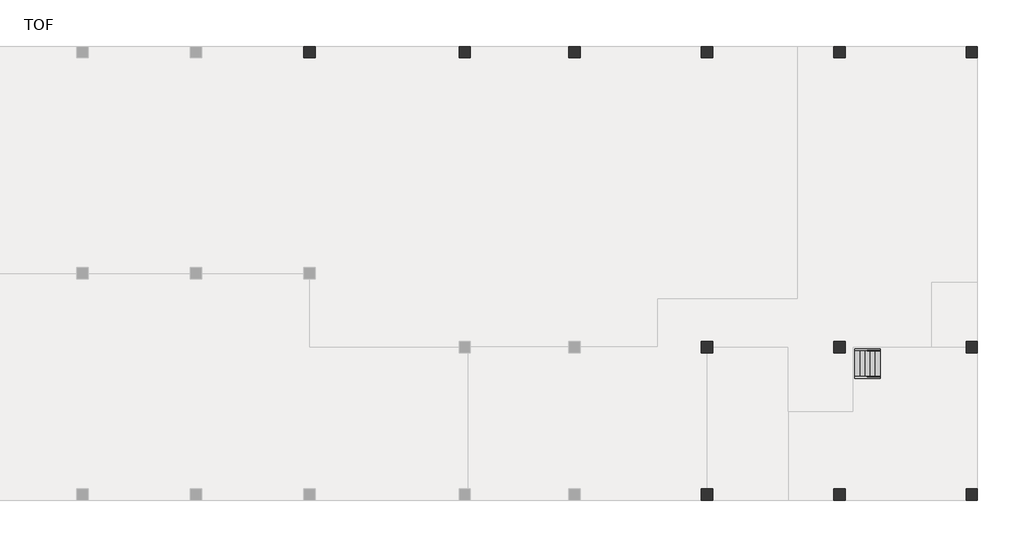
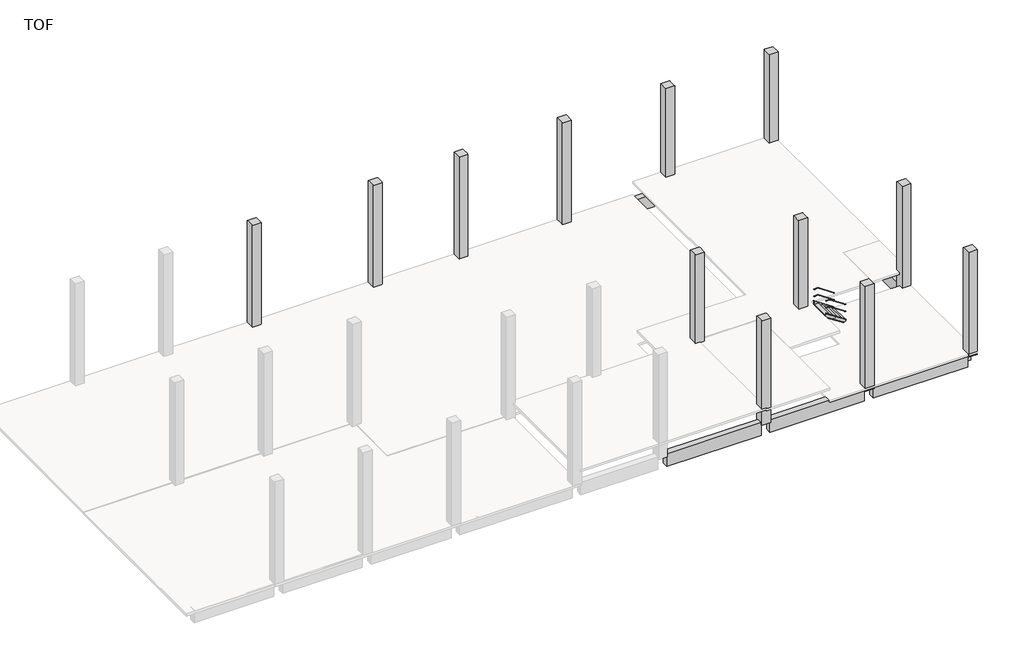
# One storey, part 2 of 2: 12 columns, 11 beams, 2 members, 2 railings, 1 stair flight.
"""IFC4 building model written with IfcOpenShell, lengths in millimetres."""

import ifcopenshell
import ifcopenshell.guid

model = None  # the IFC model being written
_history = None  # IfcOwnerHistory: only IFC2X3 demands one
_inside = {}  # id of a spatial element -> (the spatial element, [elements in it])
_under = {}  # id of a project, library or spatial element -> (it, [spatial elements below it])
_declared = {}  # id of a project -> (the project, [libraries it declares])
_typed = {}  # id of a type object -> (the type object, [elements of that type])
_made_of = {}  # id of a material, layer set ... -> (it, [elements and type objects made of it])


def new_model(schema):
    """Start an empty IFC model of exactly this schema.

    Asked for "IFC4X3", IfcOpenShell would pick the latest addendum, in which some entities
    have other attributes; the version numbers below select the first issue.
    IFC2X3 requires an IfcOwnerHistory on every rooted entity: one is made here for all.
    """
    global model, _history
    if schema == "IFC4X3":
        model = ifcopenshell.file(schema_version=(4, 3, 0, 0))
    else:
        model = ifcopenshell.file(schema=schema)
    _inside.clear()
    _under.clear()
    _declared.clear()
    _typed.clear()
    _made_of.clear()
    _history = None
    if model.schema == "IFC2X3":
        org = make("IfcOrganization", Name="unknown")
        user = make(
            "IfcPersonAndOrganization",
            ThePerson=make("IfcPerson", FamilyName="unknown"),
            TheOrganization=org,
        )
        app = make(
            "IfcApplication",
            ApplicationDeveloper=org,
            Version="unknown",
            ApplicationFullName="unknown",
            ApplicationIdentifier="unknown",
        )
        _history = make(
            "IfcOwnerHistory",
            OwningUser=user,
            OwningApplication=app,
            ChangeAction="ADDED",
            CreationDate=0,
        )
    return model


def make(cls, **values):
    """One entity of the class cls with the attributes given. An attribute that is None is left unset."""
    return model.create_entity(
        cls, **{name: value for name, value in values.items() if value is not None}
    )


def rooted(cls, **values):
    """An entity with a GlobalId (a new one), such as an element, a storey or a relation."""
    return make(cls, GlobalId=ifcopenshell.guid.new(), OwnerHistory=_history, **values)


def si_unit(unit_type, name, prefix=None):
    """IfcSIUnit, for example si_unit("LENGTHUNIT", "METRE", prefix="MILLI")."""
    return make("IfcSIUnit", UnitType=unit_type, Prefix=prefix, Name=name)


def assignment(units):
    """IfcUnitAssignment: the units of a project."""
    return None if units is None else make("IfcUnitAssignment", Units=units)


def point(xyz):
    """IfcCartesianPoint."""
    return None if xyz is None else make("IfcCartesianPoint", Coordinates=xyz)


def direction(xyz):
    """IfcDirection."""
    return None if xyz is None else make("IfcDirection", DirectionRatios=xyz)


def frame(location, z_axis=None, x_axis=None):
    """IfcAxis2Placement3D, a coordinate frame: its origin and axes. An axis left out is left unset."""
    return make(
        "IfcAxis2Placement3D",
        Location=point(location),
        Axis=direction(z_axis),
        RefDirection=direction(x_axis),
    )


def origin():
    """The frame at (0, 0, 0) with its axes left unset."""
    return frame((0.0, 0.0, 0.0))


def place(relative_to, where):
    """IfcLocalPlacement: puts the frame where relative to a parent placement (None: the world)."""
    return make(
        "IfcLocalPlacement", PlacementRelTo=relative_to, RelativePlacement=where
    )


def context(
    kind, dimensions, precision=None, world=None, true_north=None, identifier=None
):
    """IfcGeometricRepresentationContext, for example the 3D "Model" context."""
    return make(
        "IfcGeometricRepresentationContext",
        ContextIdentifier=identifier,
        ContextType=kind,
        CoordinateSpaceDimension=dimensions,
        Precision=precision,
        WorldCoordinateSystem=world,
        TrueNorth=true_north,
    )


def project(units=None, contexts=None):
    """IfcProject with its units and contexts."""
    return rooted(
        "IfcProject",
        Name="project",
        RepresentationContexts=contexts,
        UnitsInContext=assignment(units),
    )


def spatial(cls, under=None, at=None, **own):
    """A site, building, storey or space (cls), placed at a placement, below another one or the project."""
    s = rooted(cls, ObjectPlacement=at, **own)
    if under is not None:
        _under.setdefault(under.id(), (under, []))[1].append(s)
    return s


def polyline(points):
    """IfcPolyline through the points."""
    return make("IfcPolyline", Points=[point(p) for p in points])


def circle_curve(where, radius):
    """IfcCircle in the frame where."""
    return make("IfcCircle", Position=where, Radius=radius)


def ellipse_curve(where, semi_axis1, semi_axis2):
    """IfcEllipse in the frame where."""
    return make(
        "IfcEllipse", Position=where, SemiAxis1=semi_axis1, SemiAxis2=semi_axis2
    )


def outline(outer, holes=None, kind="AREA"):
    """IfcArbitraryClosedProfileDef: a profile drawn as a closed curve; with holes, ...WithVoids."""
    if holes is None:
        return make("IfcArbitraryClosedProfileDef", ProfileType=kind, OuterCurve=outer)
    return make(
        "IfcArbitraryProfileDefWithVoids",
        ProfileType=kind,
        OuterCurve=outer,
        InnerCurves=holes,
    )


def extrude(swept, where, along, depth):
    """IfcExtrudedAreaSolid: the profile swept, set in the frame where, extruded along a direction by depth."""
    return make(
        "IfcExtrudedAreaSolid",
        SweptArea=swept,
        Position=where,
        ExtrudedDirection=direction(along),
        Depth=depth,
    )


def faces_of(points, faces, orient=None, outer=None):
    """IfcFace entities. A face is a list of loops; a loop is a list of indices into points, from 0.

    orient and outer hold one flag for each loop. By default every Orientation is true, the
    first loop of a face is its IfcFaceOuterBound and the others are IfcFaceBound.
    """
    made = []
    for i, loops in enumerate(faces):
        bounds = []
        for j, loop in enumerate(loops):
            is_outer = j == 0 if outer is None else outer[i][j]
            bounds.append(
                make(
                    "IfcFaceOuterBound" if is_outer else "IfcFaceBound",
                    Bound=make("IfcPolyLoop", Polygon=[points[k] for k in loop]),
                    Orientation=True if orient is None else orient[i][j],
                )
            )
        made.append(make("IfcFace", Bounds=bounds))
    return made


def faceted_brep(points, faces, orient=None, outer=None, voids=None):
    """IfcFacetedBrep: a solid bounded by flat faces; with voids (closed shells), ...WithVoids."""
    shared = [point(p) for p in points]
    hull = make("IfcClosedShell", CfsFaces=faces_of(shared, faces, orient, outer))
    if voids is None:
        return make("IfcFacetedBrep", Outer=hull)
    return make(
        "IfcFacetedBrepWithVoids",
        Outer=hull,
        Voids=[
            make(cls, CfsFaces=faces_of(shared, fs, o, b)) for cls, fs, o, b in voids
        ],
    )


def shape(context_of_items, identifier, shape_type, items):
    """IfcShapeRepresentation: the items that make up one representation, for example the "Body"."""
    return make(
        "IfcShapeRepresentation",
        ContextOfItems=context_of_items,
        RepresentationIdentifier=identifier,
        RepresentationType=shape_type,
        Items=items,
    )


def source(mapping_origin, context_of_items, identifier, shape_type, items):
    """IfcRepresentationMap: a shape defined once, which mapped items show again and again."""
    return make(
        "IfcRepresentationMap",
        MappingOrigin=mapping_origin,
        MappedRepresentation=shape(context_of_items, identifier, shape_type, items),
    )


def transform(
    local_origin,
    x_axis=None,
    y_axis=None,
    z_axis=None,
    scale=None,
    scale2=None,
    scale3=None,
    uniform=True,
):
    """IfcCartesianTransformationOperator3D, or its non-uniform kind. x_axis, y_axis, z_axis: its Axis1, 2, 3."""
    if uniform:
        return make(
            "IfcCartesianTransformationOperator3D",
            Axis1=direction(x_axis),
            Axis2=direction(y_axis),
            LocalOrigin=point(local_origin),
            Scale=scale,
            Axis3=direction(z_axis),
        )
    return make(
        "IfcCartesianTransformationOperator3DnonUniform",
        Axis1=direction(x_axis),
        Axis2=direction(y_axis),
        LocalOrigin=point(local_origin),
        Scale=scale,
        Axis3=direction(z_axis),
        Scale2=scale2,
        Scale3=scale3,
    )


def mapped(mapping_source, mapping_target):
    """IfcMappedItem: shows the shape of a source again, moved by a transform."""
    return make(
        "IfcMappedItem", MappingSource=mapping_source, MappingTarget=mapping_target
    )


def made_of(thing, what):
    """Note that an element or type object is made of a material, layer set ...; save() writes the relation."""
    if what is not None:
        _made_of.setdefault(what.id(), (what, []))[1].append(thing)
    return thing


def element(
    cls,
    number,
    at=None,
    inside=None,
    cuts=None,
    type_object=None,
    material=None,
    context=None,
    identifier="Body",
    shape_type=None,
    held_by="IfcProductDefinitionShape",
    body=None,
    shapes=None,
    **own,
):
    """One element of the class cls, such as IfcWall. Its Tag is "e" and its number.

    at: its placement. inside: the storey or other place that contains it. cuts: it is an
    opening in that element (IfcRelVoidsElement). A single representation is given by context,
    identifier, shape_type and body (its items); several are given by shapes. held_by: the class
    of the entity that holds the representations. save() writes the other relations.
    """
    e = rooted(cls, Tag="e%d" % number, ObjectPlacement=at, **own)
    if body is not None:
        shapes = [shape(context, identifier, shape_type, body)]
    if shapes is not None:
        e.Representation = make(held_by, Representations=shapes)
    if inside is not None:
        _inside.setdefault(inside.id(), (inside, []))[1].append(e)
    if cuts is not None:
        rooted(
            "IfcRelVoidsElement", RelatingBuildingElement=cuts, RelatedOpeningElement=e
        )
    if type_object is not None:
        _typed.setdefault(type_object.id(), (type_object, []))[1].append(e)
    return made_of(e, material)


def aggregate(whole, parts):
    """IfcRelAggregates: a whole, such as a stair, and the parts it consists of."""
    return rooted("IfcRelAggregates", RelatingObject=whole, RelatedObjects=parts)


def save(model, path):
    """Write the relations noted so far, then the file.

    IfcRelAggregates (storeys below a building ...), IfcRelContainedInSpatialStructure (elements
    in a storey), IfcRelDefinesByType, IfcRelAssociatesMaterial and IfcRelDeclares: one each for
    every whole, place, type object, material and project.
    """
    for whole, parts in _under.values():
        aggregate(whole, parts)
    for where, things in _inside.values():
        rooted(
            "IfcRelContainedInSpatialStructure",
            RelatedElements=things,
            RelatingStructure=where,
        )
    for kind, things in _typed.values():
        rooted("IfcRelDefinesByType", RelatedObjects=things, RelatingType=kind)
    for what, things in _made_of.values():
        rooted("IfcRelAssociatesMaterial", RelatedObjects=things, RelatingMaterial=what)
    for by, libraries in _declared.values():
        rooted("IfcRelDeclares", RelatingContext=by, RelatedDefinitions=libraries)
    model.write(path)


def plane_surface(at):
    """IfcPlane: the flat surface through the origin of the frame at, square to its z axis."""
    return make("IfcPlane", Position=at)


def cylinder_surface(at, radius):
    """IfcCylindricalSurface: all points at the distance radius from the z axis of the frame at."""
    return make("IfcCylindricalSurface", Position=at, Radius=radius)


def advanced_brep(points, edges, surfaces, faces):
    """IfcAdvancedBrep: a solid bounded by faces that lie on surfaces and meet in shared edges.

    An edge is (start, end): straight between two places in points (the first is 0);
    or (start, end, curve); or (start, end, curve, False) where it runs against its curve.
    A face is (place in surfaces, loops), or (place, loops, False) where it looks against
    its surface's normal. A loop lists edges by number (the first is 1), with a minus sign
    where the edge is run from its end to its start. The first loop is the outer one.
    """
    corners = [point(p) for p in points]
    vertices = [make("IfcVertexPoint", VertexGeometry=c) for c in corners]
    made = []
    for start, end, *more in edges:
        made.append(
            make(
                "IfcEdgeCurve",
                EdgeStart=vertices[start],
                EdgeEnd=vertices[end],
                EdgeGeometry=more[0] if more else make("IfcPolyline", Points=[corners[start], corners[end]]),
                SameSense=more[1] if len(more) > 1 else True,
            )
        )
    hull = []
    for where, loops, *sense in faces:
        bounds = []
        for j, loop in enumerate(loops):
            ring = [make("IfcOrientedEdge", EdgeElement=made[abs(k) - 1], Orientation=k > 0) for k in loop]
            bounds.append(
                make(
                    "IfcFaceOuterBound" if j == 0 else "IfcFaceBound",
                    Bound=make("IfcEdgeLoop", EdgeList=ring),
                    Orientation=True,
                )
            )
        hull.append(make("IfcAdvancedFace", Bounds=bounds, FaceSurface=surfaces[where], SameSense=sense[0] if sense else True))
    return make("IfcAdvancedBrep", Outer=make("IfcClosedShell", CfsFaces=hull))


def railing_36ed9c91(model_context):
    return source(origin(), model_context, "Body", "AdvancedBrep", [
        advanced_brep(
        [(48078.2332408, 8219.6306666, 910.5875748), (48078.2332408, 8249.6306666, 910.5875748), (46993.7216539, 8219.6306666, 1627.8571429), (46993.7216539, 8249.6306666, 1627.8571429), (46728.2332408, 8219.6306666, 1627.8571429), (46728.2332408, 8249.6306666, 1627.8571429)],
        [
            (0, 1, ellipse_curve(frame((48078.2332408, 8234.6306666, 910.5875748), z_axis=(1.0, 0.0, 0.0), x_axis=(0.0, 0.0, -1.0)), 17.9838538, 15.0)),
            (1, 0, ellipse_curve(frame((48078.2332408, 8234.6306666, 910.5875748), z_axis=(1.0, 0.0, 0.0), x_axis=(0.0, 0.0, -1.0)), 17.9838538, 15.0)),
            (0, 2),
            (2, 3, ellipse_curve(frame((46993.7216539, 8234.6306666, 1627.8571429), z_axis=(0.9576224501515418, 0.0, -0.28802646226650325), x_axis=(-0.288026462266502, 0.0, -0.9576224501515423)), 15.6637932, 15.0)),
            (3, 1),
            (3, 2, ellipse_curve(frame((46993.7216539, 8234.6306666, 1627.8571429), z_axis=(0.9576224501515418, 0.0, -0.28802646226650325), x_axis=(-0.288026462266502, 0.0, -0.9576224501515423)), 15.6637932, 15.0)),
            (4, 5, circle_curve(frame((46728.2332408, 8234.6306666, 1627.8571429), z_axis=(-1.0, 0.0, 0.0), x_axis=(0.0, 1.0, 0.0)), 15.0)),
            (5, 4, circle_curve(frame((46728.2332408, 8234.6306666, 1627.8571429), z_axis=(-1.0, 0.0, 0.0), x_axis=(0.0, 1.0, 0.0)), 15.0)),
            (2, 4),
            (5, 3),
        ],
        [
            plane_surface(frame((48078.2332408, 8234.6306666, 928.5714286), z_axis=(1.0, 0.0, 0.0), x_axis=(0.0, -1.0, 0.0))),
            cylinder_surface(frame((48069.9586226, 8234.6306666, 916.0602059), z_axis=(0.8340815140684851, 0.0, -0.5516412130082591), x_axis=(0.0, 1.0, 0.0)), 15.0),
            plane_surface(frame((46728.2332408, 8234.6306666, 1642.8571429), z_axis=(-1.0, 0.0, 0.0), x_axis=(0.0, -1.0, 0.0))),
            cylinder_surface(frame((46998.2332408, 8234.6306666, 1627.8571429), z_axis=(1.0, 0.0, 0.0), x_axis=(0.0, 1.0, 0.0)), 15.0),
        ],
        [
            (0, [[1, 2]]),
            (1, [[-1, 3, 4, 5]]),
            (1, [[-2, -5, 6, -3]]),
            (2, [[7, 8]]),
            (3, [[-4, 9, -8, 10]]),
            (3, [[-6, -10, -7, -9]]),
        ],
    ),
        advanced_brep(
        [(48078.2332408, 8219.6306666, 1410.5875748), (48078.2332408, 8249.6306666, 1410.5875748), (46993.7216539, 8219.6306666, 2127.8571429), (46993.7216539, 8249.6306666, 2127.8571429), (46728.2332408, 8219.6306666, 2127.8571429), (46728.2332408, 8249.6306666, 2127.8571429)],
        [
            (0, 1, ellipse_curve(frame((48078.2332408, 8234.6306666, 1410.5875748), z_axis=(1.0, 0.0, 0.0), x_axis=(0.0, 0.0, -1.0)), 17.9838538, 15.0)),
            (1, 0, ellipse_curve(frame((48078.2332408, 8234.6306666, 1410.5875748), z_axis=(1.0, 0.0, 0.0), x_axis=(0.0, 0.0, -1.0)), 17.9838538, 15.0)),
            (0, 2),
            (2, 3, ellipse_curve(frame((46993.7216539, 8234.6306666, 2127.8571429), z_axis=(0.9576224501515418, 0.0, -0.28802646226650325), x_axis=(-0.288026462266502, 0.0, -0.9576224501515423)), 15.6637932, 15.0)),
            (3, 1),
            (3, 2, ellipse_curve(frame((46993.7216539, 8234.6306666, 2127.8571429), z_axis=(0.9576224501515418, 0.0, -0.28802646226650325), x_axis=(-0.288026462266502, 0.0, -0.9576224501515423)), 15.6637932, 15.0)),
            (4, 5, circle_curve(frame((46728.2332408, 8234.6306666, 2127.8571429), z_axis=(-1.0, 0.0, 0.0), x_axis=(0.0, 1.0, 0.0)), 15.0)),
            (5, 4, circle_curve(frame((46728.2332408, 8234.6306666, 2127.8571429), z_axis=(-1.0, 0.0, 0.0), x_axis=(0.0, 1.0, 0.0)), 15.0)),
            (2, 4),
            (5, 3),
        ],
        [
            plane_surface(frame((48078.2332408, 8234.6306666, 1428.5714286), z_axis=(1.0, 0.0, 0.0), x_axis=(0.0, -1.0, 0.0))),
            cylinder_surface(frame((48069.9586226, 8234.6306666, 1416.0602059), z_axis=(0.8340815140684851, 0.0, -0.5516412130082591), x_axis=(0.0, 1.0, 0.0)), 15.0),
            plane_surface(frame((46728.2332408, 8234.6306666, 2142.8571429), z_axis=(-1.0, 0.0, 0.0), x_axis=(0.0, -1.0, 0.0))),
            cylinder_surface(frame((46998.2332408, 8234.6306666, 2127.8571429), z_axis=(1.0, 0.0, 0.0), x_axis=(0.0, 1.0, 0.0)), 15.0),
        ],
        [
            (0, [[1, 2]]),
            (1, [[-1, 3, 4, 5]]),
            (1, [[-2, -5, 6, -3]]),
            (2, [[7, 8]]),
            (3, [[-4, 9, -8, 10]]),
            (3, [[-6, -10, -7, -9]]),
        ],
    ),
    ])


def railing_d88b3958(model_context):
    return source(origin(), model_context, "Body", "AdvancedBrep", [
        advanced_brep(
        [(48078.2332408, 6875.4306666, 910.5875748), (48078.2332408, 6845.4306666, 910.5875748), (46993.7216539, 6875.4306666, 1627.8571429), (46993.7216539, 6845.4306666, 1627.8571429), (46728.2332408, 6875.4306666, 1627.8571429), (46728.2332408, 6845.4306666, 1627.8571429)],
        [
            (0, 1, ellipse_curve(frame((48078.2332408, 6860.4306666, 910.5875748), z_axis=(1.0, 0.0, 0.0), x_axis=(0.0, 0.0, -1.0)), 17.9838538, 15.0)),
            (1, 0, ellipse_curve(frame((48078.2332408, 6860.4306666, 910.5875748), z_axis=(1.0, 0.0, 0.0), x_axis=(0.0, 0.0, -1.0)), 17.9838538, 15.0)),
            (0, 2),
            (2, 3, ellipse_curve(frame((46993.7216539, 6860.4306666, 1627.8571429), z_axis=(0.9576224501515418, 0.0, -0.28802646226650325), x_axis=(-0.288026462266502, 0.0, -0.9576224501515423)), 15.6637932, 15.0)),
            (3, 1),
            (3, 2, ellipse_curve(frame((46993.7216539, 6860.4306666, 1627.8571429), z_axis=(0.9576224501515418, 0.0, -0.28802646226650325), x_axis=(-0.288026462266502, 0.0, -0.9576224501515423)), 15.6637932, 15.0)),
            (4, 5, circle_curve(frame((46728.2332408, 6860.4306666, 1627.8571429), z_axis=(-1.0, 0.0, 0.0), x_axis=(0.0, -1.0, 0.0)), 15.0)),
            (5, 4, circle_curve(frame((46728.2332408, 6860.4306666, 1627.8571429), z_axis=(-1.0, 0.0, 0.0), x_axis=(0.0, -1.0, 0.0)), 15.0)),
            (2, 4),
            (5, 3),
        ],
        [
            plane_surface(frame((48078.2332408, 6860.4306666, 928.5714286), z_axis=(1.0, 0.0, 0.0), x_axis=(0.0, -1.0, 0.0))),
            cylinder_surface(frame((48069.9586226, 6860.4306666, 916.0602059), z_axis=(0.8340815140684851, 0.0, -0.5516412130082591), x_axis=(0.0, -1.0, 0.0)), 15.0),
            plane_surface(frame((46728.2332408, 6860.4306666, 1642.8571429), z_axis=(-1.0, 0.0, 0.0), x_axis=(0.0, -1.0, 0.0))),
            cylinder_surface(frame((46998.2332408, 6860.4306666, 1627.8571429), z_axis=(1.0, 0.0, 0.0), x_axis=(0.0, -1.0, 0.0)), 15.0),
        ],
        [
            (0, [[1, 2]]),
            (1, [[-1, 3, 4, 5]]),
            (1, [[-2, -5, 6, -3]]),
            (2, [[7, 8]]),
            (3, [[-4, 9, -8, 10]]),
            (3, [[-6, -10, -7, -9]]),
        ],
    ),
        advanced_brep(
        [(48078.2332408, 6875.4306666, 1410.5875748), (48078.2332408, 6845.4306666, 1410.5875748), (46993.7216539, 6875.4306666, 2127.8571429), (46993.7216539, 6845.4306666, 2127.8571429), (46728.2332408, 6875.4306666, 2127.8571429), (46728.2332408, 6845.4306666, 2127.8571429)],
        [
            (0, 1, ellipse_curve(frame((48078.2332408, 6860.4306666, 1410.5875748), z_axis=(1.0, 0.0, 0.0), x_axis=(0.0, 0.0, -1.0)), 17.9838538, 15.0)),
            (1, 0, ellipse_curve(frame((48078.2332408, 6860.4306666, 1410.5875748), z_axis=(1.0, 0.0, 0.0), x_axis=(0.0, 0.0, -1.0)), 17.9838538, 15.0)),
            (0, 2),
            (2, 3, ellipse_curve(frame((46993.7216539, 6860.4306666, 2127.8571429), z_axis=(0.9576224501515418, 0.0, -0.28802646226650325), x_axis=(-0.288026462266502, 0.0, -0.9576224501515423)), 15.6637932, 15.0)),
            (3, 1),
            (3, 2, ellipse_curve(frame((46993.7216539, 6860.4306666, 2127.8571429), z_axis=(0.9576224501515418, 0.0, -0.28802646226650325), x_axis=(-0.288026462266502, 0.0, -0.9576224501515423)), 15.6637932, 15.0)),
            (4, 5, circle_curve(frame((46728.2332408, 6860.4306666, 2127.8571429), z_axis=(-1.0, 0.0, 0.0), x_axis=(0.0, -1.0, 0.0)), 15.0)),
            (5, 4, circle_curve(frame((46728.2332408, 6860.4306666, 2127.8571429), z_axis=(-1.0, 0.0, 0.0), x_axis=(0.0, -1.0, 0.0)), 15.0)),
            (2, 4),
            (5, 3),
        ],
        [
            plane_surface(frame((48078.2332408, 6860.4306666, 1428.5714286), z_axis=(1.0, 0.0, 0.0), x_axis=(0.0, -1.0, 0.0))),
            cylinder_surface(frame((48069.9586226, 6860.4306666, 1416.0602059), z_axis=(0.8340815140684851, 0.0, -0.5516412130082591), x_axis=(0.0, -1.0, 0.0)), 15.0),
            plane_surface(frame((46728.2332408, 6860.4306666, 2142.8571429), z_axis=(-1.0, 0.0, 0.0), x_axis=(0.0, -1.0, 0.0))),
            cylinder_surface(frame((46998.2332408, 6860.4306666, 2127.8571429), z_axis=(1.0, 0.0, 0.0), x_axis=(0.0, -1.0, 0.0)), 15.0),
        ],
        [
            (0, [[1, 2]]),
            (1, [[-1, 3, 4, 5]]),
            (1, [[-2, -5, 6, -3]]),
            (2, [[7, 8]]),
            (3, [[-4, 9, -8, 10]]),
            (3, [[-6, -10, -7, -9]]),
        ],
    ),
    ])


def stair_flight_4e27faa5(model_context):
    return source(origin(), model_context, "Body", "SweptSolid", [
        extrude(outline(polyline([(47808.2332408, 6860.0306666), (47808.2332408, 8235.0306666), (48078.2332408, 8235.0306666), (48078.2332408, 6860.0306666), (47808.2332408, 6860.0306666)])), frame((0.0, 0.0, 296.5714286), z_axis=(0.0, 0.0, 1.0), x_axis=(1.0, 0.0, 0.0)), (0.0, 0.0, 1.0), 32.0),
        extrude(outline(polyline([(47538.2332408, 6860.0306666), (47538.2332408, 8235.0306666), (47808.2332408, 8235.0306666), (47808.2332408, 6860.0306666), (47538.2332408, 6860.0306666)])), frame((0.0, 0.0, 475.1428571), z_axis=(0.0, 0.0, 1.0), x_axis=(1.0, 0.0, 0.0)), (0.0, 0.0, 1.0), 32.0),
        extrude(outline(polyline([(47268.2332408, 6860.0306666), (47268.2332408, 8235.0306666), (47538.2332408, 8235.0306666), (47538.2332408, 6860.0306666), (47268.2332408, 6860.0306666)])), frame((0.0, 0.0, 653.7142857), z_axis=(0.0, 0.0, 1.0), x_axis=(1.0, 0.0, 0.0)), (0.0, 0.0, 1.0), 32.0),
        extrude(outline(polyline([(46998.2332408, 6860.0306666), (46998.2332408, 8235.0306666), (47268.2332408, 8235.0306666), (47268.2332408, 6860.0306666), (46998.2332408, 6860.0306666)])), frame((0.0, 0.0, 832.2857143), z_axis=(0.0, 0.0, 1.0), x_axis=(1.0, 0.0, 0.0)), (0.0, 0.0, 1.0), 32.0),
        extrude(outline(polyline([(46728.2332408, 6860.0306666), (46728.2332408, 8235.0306666), (46998.2332408, 8235.0306666), (46998.2332408, 6860.0306666), (46728.2332408, 6860.0306666)])), frame((0.0, 0.0, 1010.8571429), z_axis=(0.0, 0.0, 1.0), x_axis=(1.0, 0.0, 0.0)), (0.0, 0.0, 1.0), 32.0),
    ])


model = new_model("IFC4")

# Units and contexts
model_context = context("Model", 3, world=origin())
ifc_project = project(units=[si_unit("LENGTHUNIT", "METRE", prefix="MILLI")], contexts=[model_context])

# Site, building, storey
site = spatial("IfcSite", under=ifc_project)
building = spatial("IfcBuilding", under=site)
storey = spatial("IfcBuildingStorey", under=building, Name="TOF", Elevation=150.0)

# Beams
placement = place(None, origin())
element("IfcBeam", 1, ObjectType="RC Beam_Rectangular : H_SB_ACB_B400xH900", at=placement, inside=storey, context=model_context, shape_type="SweptSolid", body=[
    extrude(outline(polyline([(52724.7, 23716.5208589), (53124.7, 23716.5208589), (53124.7, 18966.5208589), (52724.7, 18966.5208589), (52724.7, 23716.5208589)])), frame((0.0, 0.0, -750.0), z_axis=(0.0, 0.0, 1.0), x_axis=(1.0, 0.0, 0.0)), (0.0, 0.0, 1.0), 900.0),
    extrude(outline(polyline([(53124.7, 8716.5208589), (52724.7, 8716.5208589), (52724.7, 18366.5208589), (53124.7, 18366.5208589), (53124.7, 8716.5208589)])), frame((0.0, 0.0, -750.0), z_axis=(0.0, 0.0, 1.0), x_axis=(1.0, 0.0, 0.0)), (0.0, 0.0, 1.0), 900.0),
])
element("IfcBeam", 2, ObjectType="RC Beam_Rectangular : H_SB_ACB_B400xH900", at=placement, inside=storey, context=model_context, shape_type="SweptSolid", body=[
    extrude(outline(polyline([(52724.7, 8116.5208589), (53124.7, 8116.5208589), (53124.7, 916.5208589), (52724.7, 916.5208589), (52724.7, 8116.5208589)])), frame((0.0, 0.0, -750.0), z_axis=(0.0, 0.0, 1.0), x_axis=(1.0, 0.0, 0.0)), (0.0, 0.0, 1.0), 900.0),
])
element("IfcBeam", 3, ObjectType="RC Beam_Rectangular : H_SB_ACB_B400xH900", at=placement, inside=storey, context=model_context, shape_type="SweptSolid", body=[
    extrude(outline(polyline([(12224.7, 23816.5208589), (12224.7, 24216.5208589), (17624.7, 24216.5208589), (17624.7, 23816.5208589), (12224.7, 23816.5208589)])), frame((0.0, 0.0, -750.0), z_axis=(0.0, 0.0, 1.0), x_axis=(1.0, 0.0, 0.0)), (0.0, 0.0, 1.0), 900.0),
])
element("IfcBeam", 4, ObjectType="RC Beam_Rectangular : H_SB_ACB_B400xH900", at=placement, inside=storey, context=model_context, shape_type="SweptSolid", body=[
    extrude(outline(polyline([(18224.7, 23816.5208589), (18224.7, 24216.5208589), (25824.7, 24216.5208589), (25824.7, 23816.5208589), (18224.7, 23816.5208589)])), frame((0.0, 0.0, -750.0), z_axis=(0.0, 0.0, 1.0), x_axis=(1.0, 0.0, 0.0)), (0.0, 0.0, 1.0), 900.0),
])
element("IfcBeam", 5, ObjectType="RC Beam_Rectangular : H_SB_ACB_B400xH900", at=placement, inside=storey, context=model_context, shape_type="SweptSolid", body=[
    extrude(outline(polyline([(26424.7, 23816.5208589), (26424.7, 24216.5208589), (31624.7, 24216.5208589), (31624.7, 23816.5208589), (26424.7, 23816.5208589)])), frame((0.0, 0.0, -750.0), z_axis=(0.0, 0.0, 1.0), x_axis=(1.0, 0.0, 0.0)), (0.0, 0.0, 1.0), 900.0),
])
element("IfcBeam", 6, ObjectType="RC Beam_Rectangular : H_SB_ACB_B400xH900", at=placement, inside=storey, context=model_context, shape_type="SweptSolid", body=[
    extrude(outline(polyline([(32224.7, 23816.5208589), (32224.7, 24216.5208589), (38624.7, 24216.5208589), (38624.7, 23816.5208589), (32224.7, 23816.5208589)])), frame((0.0, 0.0, -750.0), z_axis=(0.0, 0.0, 1.0), x_axis=(1.0, 0.0, 0.0)), (0.0, 0.0, 1.0), 900.0),
])
element("IfcBeam", 7, ObjectType="RC Beam_Rectangular : H_SB_ACB_B400xH900", at=placement, inside=storey, context=model_context, shape_type="SweptSolid", body=[
    extrude(outline(polyline([(39224.7, 23816.5208589), (39224.7, 24216.5208589), (45624.7, 24216.5208589), (45624.7, 23816.5208589), (39224.7, 23816.5208589)])), frame((0.0, 0.0, -750.0), z_axis=(0.0, 0.0, 1.0), x_axis=(1.0, 0.0, 0.0)), (0.0, 0.0, 1.0), 900.0),
])
element("IfcBeam", 8, ObjectType="RC Beam_Rectangular : H_SB_ACB_B400xH900", at=placement, inside=storey, context=model_context, shape_type="SweptSolid", body=[
    extrude(outline(polyline([(46224.7, 23816.5208589), (46224.7, 24216.5208589), (52624.7, 24216.5208589), (52624.7, 23816.5208589), (46224.7, 23816.5208589)])), frame((0.0, 0.0, -750.0), z_axis=(0.0, 0.0, 1.0), x_axis=(1.0, 0.0, 0.0)), (0.0, 0.0, 1.0), 900.0),
])
element("IfcBeam", 9, ObjectType="RC Beam_Rectangular : H_SB_ACB_B400xH900", at=placement, inside=storey, context=model_context, shape_type="SweptSolid", body=[
    extrude(outline(polyline([(32224.7, 416.5208589), (32224.7, 816.5208589), (38624.7, 816.5208589), (38624.7, 416.5208589), (32224.7, 416.5208589)])), frame((0.0, 0.0, -750.0), z_axis=(0.0, 0.0, 1.0), x_axis=(1.0, 0.0, 0.0)), (0.0, 0.0, 1.0), 900.0),
])
element("IfcBeam", 10, ObjectType="RC Beam_Rectangular : H_SB_ACB_B400xH900", at=placement, inside=storey, context=model_context, shape_type="SweptSolid", body=[
    extrude(outline(polyline([(39224.7, 416.5208589), (39224.7, 816.5208589), (45624.7, 816.5208589), (45624.7, 416.5208589), (39224.7, 416.5208589)])), frame((0.0, 0.0, -750.0), z_axis=(0.0, 0.0, 1.0), x_axis=(1.0, 0.0, 0.0)), (0.0, 0.0, 1.0), 900.0),
])
element("IfcBeam", 11, ObjectType="RC Beam_Rectangular : H_SB_ACB_B400xH900", at=placement, inside=storey, context=model_context, shape_type="SweptSolid", body=[
    extrude(outline(polyline([(46224.7, 416.5208589), (46224.7, 816.5208589), (52624.7, 816.5208589), (52624.7, 416.5208589), (46224.7, 416.5208589)])), frame((0.0, 0.0, -750.0), z_axis=(0.0, 0.0, 1.0), x_axis=(1.0, 0.0, 0.0)), (0.0, 0.0, 1.0), 900.0),
])

# Columns
element("IfcColumn", 12, ObjectType="RC_Column_Rectangular : H_SC_ACC_W600xL600", at=placement, inside=storey, context=model_context, shape_type="Brep", body=[
    faceted_brep([(18224.7, 24316.5208589, 0.0), (18224.7, 23716.5208589, 0.0), (17624.7, 23716.5208589, 0.0), (17624.7, 24316.5208589, 0.0), (18224.7, 23716.5208589, 50.0), (18224.7, 24316.5208589, 50.0), (17624.7, 24316.5208589, 50.0), (17624.7, 23716.5208589, 50.0)], [[[0, 1, 2, 3]], [[4, 5, 6, 7]], [[1, 0, 5, 4]], [[2, 1, 4, 7]], [[3, 2, 7, 6]], [[0, 3, 6, 5]]]),
    faceted_brep([(18224.7, 24316.5208589, 7500.0), (18224.7, 24216.5208589, 7500.0), (18224.7, 23816.5208589, 7500.0), (18224.7, 23716.5208589, 7500.0), (18224.7, 23716.5208589, 200.0), (18224.7, 24316.5208589, 200.0), (18124.7, 23716.5208589, 7500.0), (17724.7, 23716.5208589, 7500.0), (17624.7, 23716.5208589, 7500.0), (17624.7, 23716.5208589, 200.0), (17624.7, 23816.5208589, 7500.0), (17624.7, 24216.5208589, 7500.0), (17624.7, 24316.5208589, 7500.0), (17624.7, 24316.5208589, 200.0), (17724.7, 24316.5208589, 7500.0), (18124.7, 24316.5208589, 7500.0)], [[[0, 1, 2, 3, 4, 5]], [[3, 6, 7, 8, 9, 4]], [[8, 10, 11, 12, 13, 9]], [[12, 14, 15, 0, 5, 13]], [[3, 2, 1, 0, 15, 14, 12, 11, 10, 8, 7, 6]], [[5, 4, 9, 13]]]),
])
element("IfcColumn", 13, ObjectType="RC_Column_Rectangular : H_SC_ACC_W600xL600", at=placement, inside=storey, context=model_context, shape_type="Brep", body=[
    faceted_brep([(26424.7, 24316.5208589, 0.0), (26424.7, 23716.5208589, 0.0), (25824.7, 23716.5208589, 0.0), (25824.7, 24316.5208589, 0.0), (26424.7, 23716.5208589, 50.0), (26424.7, 24316.5208589, 50.0), (25824.7, 24316.5208589, 50.0), (25824.7, 23716.5208589, 50.0)], [[[0, 1, 2, 3]], [[4, 5, 6, 7]], [[1, 0, 5, 4]], [[2, 1, 4, 7]], [[3, 2, 7, 6]], [[0, 3, 6, 5]]]),
    faceted_brep([(26424.7, 24316.5208589, 7500.0), (26424.7, 24216.5208589, 7500.0), (26424.7, 23816.5208589, 7500.0), (26424.7, 23716.5208589, 7500.0), (26424.7, 23716.5208589, 200.0), (26424.7, 24316.5208589, 200.0), (26324.7, 23716.5208589, 7500.0), (25924.7, 23716.5208589, 7500.0), (25824.7, 23716.5208589, 7500.0), (25824.7, 23716.5208589, 200.0), (25824.7, 23816.5208589, 7500.0), (25824.7, 24216.5208589, 7500.0), (25824.7, 24316.5208589, 7500.0), (25824.7, 24316.5208589, 200.0), (25924.7, 24316.5208589, 7500.0), (26324.7, 24316.5208589, 7500.0)], [[[0, 1, 2, 3, 4, 5]], [[3, 6, 7, 8, 9, 4]], [[8, 10, 11, 12, 13, 9]], [[12, 14, 15, 0, 5, 13]], [[3, 2, 1, 0, 15, 14, 12, 11, 10, 8, 7, 6]], [[5, 4, 9, 13]]]),
])
element("IfcColumn", 14, ObjectType="RC_Column_Rectangular : H_SC_ACC_W600xL600", at=placement, inside=storey, context=model_context, shape_type="Brep", body=[
    faceted_brep([(32224.7, 24316.5208589, 0.0), (32224.7, 23716.5208589, 0.0), (31624.7, 23716.5208589, 0.0), (31624.7, 24316.5208589, 0.0), (32224.7, 23716.5208589, 50.0), (32224.7, 24316.5208589, 50.0), (31624.7, 24316.5208589, 50.0), (31624.7, 23716.5208589, 50.0)], [[[0, 1, 2, 3]], [[4, 5, 6, 7]], [[1, 0, 5, 4]], [[2, 1, 4, 7]], [[3, 2, 7, 6]], [[0, 3, 6, 5]]]),
    faceted_brep([(32224.7, 24316.5208589, 7500.0), (32224.7, 24216.5208589, 7500.0), (32224.7, 23816.5208589, 7500.0), (32224.7, 23716.5208589, 7500.0), (32224.7, 23716.5208589, 200.0), (32224.7, 24316.5208589, 200.0), (32124.7, 23716.5208589, 7500.0), (31724.7, 23716.5208589, 7500.0), (31624.7, 23716.5208589, 7500.0), (31624.7, 23716.5208589, 200.0), (31624.7, 23816.5208589, 7500.0), (31624.7, 24216.5208589, 7500.0), (31624.7, 24316.5208589, 7500.0), (31624.7, 24316.5208589, 200.0), (31724.7, 24316.5208589, 7500.0), (32124.7, 24316.5208589, 7500.0)], [[[0, 1, 2, 3, 4, 5]], [[3, 6, 7, 8, 9, 4]], [[8, 10, 11, 12, 13, 9]], [[12, 14, 15, 0, 5, 13]], [[3, 2, 1, 0, 15, 14, 12, 11, 10, 8, 7, 6]], [[5, 4, 9, 13]]]),
])
element("IfcColumn", 15, ObjectType="RC_Column_Rectangular : H_SC_ACC_W600xL600", at=placement, inside=storey, context=model_context, shape_type="Brep", body=[
    faceted_brep([(39224.7, 24316.5208589, 0.0), (39224.7, 23716.5208589, 0.0), (38624.7, 23716.5208589, 0.0), (38624.7, 24316.5208589, 0.0), (39224.7, 23716.5208589, 50.0), (39224.7, 24316.5208589, 50.0), (38624.7, 24316.5208589, 50.0), (38624.7, 23716.5208589, 50.0)], [[[0, 1, 2, 3]], [[4, 5, 6, 7]], [[1, 0, 5, 4]], [[2, 1, 4, 7]], [[3, 2, 7, 6]], [[0, 3, 6, 5]]]),
    faceted_brep([(39224.7, 24316.5208589, 7500.0), (39224.7, 24216.5208589, 7500.0), (39224.7, 23816.5208589, 7500.0), (39224.7, 23716.5208589, 7500.0), (39224.7, 23716.5208589, 200.0), (39224.7, 24316.5208589, 200.0), (39124.7, 23716.5208589, 7500.0), (38724.7, 23716.5208589, 7500.0), (38624.7, 23716.5208589, 7500.0), (38624.7, 23716.5208589, 200.0), (38624.7, 23816.5208589, 7500.0), (38624.7, 24216.5208589, 7500.0), (38624.7, 24316.5208589, 7500.0), (38624.7, 24316.5208589, 200.0), (38724.7, 24316.5208589, 7500.0), (39124.7, 24316.5208589, 7500.0)], [[[0, 1, 2, 3, 4, 5]], [[3, 6, 7, 8, 9, 4]], [[8, 10, 11, 12, 13, 9]], [[12, 14, 15, 0, 5, 13]], [[3, 2, 1, 0, 15, 14, 12, 11, 10, 8, 7, 6]], [[5, 4, 9, 13]]]),
])
element("IfcColumn", 16, ObjectType="RC_Column_Rectangular : H_SC_ACC_W600xL600", at=placement, inside=storey, context=model_context, shape_type="Brep", body=[
    faceted_brep([(46224.7, 24316.5208589, 0.0), (46224.7, 23716.5208589, 0.0), (45624.7, 23716.5208589, 0.0), (45624.7, 24316.5208589, 0.0), (46224.7, 24316.5208589, 7500.0), (46224.7, 24216.5208589, 7500.0), (46224.7, 23816.5208589, 7500.0), (46224.7, 23716.5208589, 7500.0), (46124.7, 23716.5208589, 7500.0), (45724.7, 23716.5208589, 7500.0), (45624.7, 23716.5208589, 7500.0), (45624.7, 23816.5208589, 7500.0), (45624.7, 24216.5208589, 7500.0), (45624.7, 24316.5208589, 7500.0), (45724.7, 24316.5208589, 7500.0), (46124.7, 24316.5208589, 7500.0)], [[[0, 1, 2, 3]], [[4, 5, 6, 7, 1, 0]], [[7, 8, 9, 10, 2, 1]], [[10, 11, 12, 13, 3, 2]], [[13, 14, 15, 4, 0, 3]], [[4, 15, 14, 13, 12, 11, 10, 9, 8, 7, 6, 5]]]),
])
element("IfcColumn", 17, ObjectType="RC_Column_Rectangular : H_SC_ACC_W600xL600", at=placement, inside=storey, context=model_context, shape_type="Brep", body=[
    faceted_brep([(53224.7, 24316.5208589, 0.0), (53224.7, 23716.5208589, 0.0), (52624.7, 23716.5208589, 0.0), (52624.7, 24316.5208589, 0.0), (53224.7, 24316.5208589, 7500.0), (53224.7, 23716.5208589, 7500.0), (53124.7, 23716.5208589, 7500.0), (52724.7, 23716.5208589, 7500.0), (52624.7, 23716.5208589, 7500.0), (52624.7, 23816.5208589, 7500.0), (52624.7, 24216.5208589, 7500.0), (52624.7, 24316.5208589, 7500.0), (52724.7, 24316.5208589, 7500.0), (53124.7, 24316.5208589, 7500.0)], [[[0, 1, 2, 3]], [[4, 5, 1, 0]], [[5, 6, 7, 8, 2, 1]], [[8, 9, 10, 11, 3, 2]], [[11, 12, 13, 4, 0, 3]], [[4, 13, 12, 11, 10, 9, 8, 7, 6, 5]]]),
])
element("IfcColumn", 18, ObjectType="RC_Column_Rectangular : H_SC_ACC_W600xL600", at=placement, inside=storey, context=model_context, shape_type="Brep", body=[
    faceted_brep([(39224.7, 8716.5208589, 0.0), (39224.7, 8116.5208589, 0.0), (38624.7, 8116.5208589, 0.0), (38624.7, 8716.5208589, 0.0), (39224.7, 8716.5208589, 7500.0), (39224.7, 8616.5208589, 7500.0), (39224.7, 8216.5208589, 7500.0), (39224.7, 8116.5208589, 7500.0), (39124.7, 8116.5208589, 7500.0), (38724.7, 8116.5208589, 7500.0), (38624.7, 8116.5208589, 7500.0), (38624.7, 8216.5208589, 7500.0), (38624.7, 8616.5208589, 7500.0), (38624.7, 8716.5208589, 7500.0), (38724.7, 8716.5208589, 7500.0), (39124.7, 8716.5208589, 7500.0)], [[[0, 1, 2, 3]], [[1, 0, 4, 5, 6, 7]], [[2, 1, 7, 8, 9, 10]], [[3, 2, 10, 11, 12, 13]], [[0, 3, 13, 14, 15, 4]], [[7, 6, 5, 4, 15, 14, 13, 12, 11, 10, 9, 8]]]),
])
element("IfcColumn", 19, ObjectType="RC_Column_Rectangular : H_SC_ACC_W600xL600", at=placement, inside=storey, context=model_context, shape_type="Brep", body=[
    faceted_brep([(46224.7, 8716.5208589, 0.0), (46224.7, 8116.5208589, 0.0), (45624.7, 8116.5208589, 0.0), (45624.7, 8716.5208589, 0.0), (46224.7, 8716.5208589, 7500.0), (46224.7, 8616.5208589, 7500.0), (46224.7, 8216.5208589, 7500.0), (46224.7, 8116.5208589, 7500.0), (46124.7, 8116.5208589, 7500.0), (45724.7, 8116.5208589, 7500.0), (45624.7, 8116.5208589, 7500.0), (45624.7, 8216.5208589, 7500.0), (45624.7, 8616.5208589, 7500.0), (45624.7, 8716.5208589, 7500.0), (45724.7, 8716.5208589, 7500.0), (46124.7, 8716.5208589, 7500.0)], [[[0, 1, 2, 3]], [[4, 5, 6, 7, 1, 0]], [[7, 8, 9, 10, 2, 1]], [[10, 11, 12, 13, 3, 2]], [[13, 14, 15, 4, 0, 3]], [[4, 15, 14, 13, 12, 11, 10, 9, 8, 7, 6, 5]]]),
])
element("IfcColumn", 20, ObjectType="RC_Column_Rectangular : H_SC_ACC_W600xL600", at=placement, inside=storey, context=model_context, shape_type="Brep", body=[
    faceted_brep([(53224.7, 8716.5208589, 0.0), (53224.7, 8116.5208589, 0.0), (52624.7, 8116.5208589, 0.0), (52624.7, 8716.5208589, 0.0), (53224.7, 8716.5208589, 7500.0), (53224.7, 8116.5208589, 7500.0), (53124.7, 8116.5208589, 7500.0), (52724.7, 8116.5208589, 7500.0), (52624.7, 8116.5208589, 7500.0), (52624.7, 8216.5208589, 7500.0), (52624.7, 8616.5208589, 7500.0), (52624.7, 8716.5208589, 7500.0), (52724.7, 8716.5208589, 7500.0), (53124.7, 8716.5208589, 7500.0)], [[[0, 1, 2, 3]], [[4, 5, 1, 0]], [[5, 6, 7, 8, 2, 1]], [[8, 9, 10, 11, 3, 2]], [[11, 12, 13, 4, 0, 3]], [[4, 13, 12, 11, 10, 9, 8, 7, 6, 5]]]),
])
element("IfcColumn", 21, ObjectType="RC_Column_Rectangular : H_SC_ACC_W600xL600", at=placement, inside=storey, context=model_context, shape_type="Brep", body=[
    faceted_brep([(39224.7, 916.5208589, 0.0), (39224.7, 316.5208589, 0.0), (38624.7, 316.5208589, 0.0), (38624.7, 916.5208589, 0.0), (39224.7, 916.5208589, 7500.0), (39224.7, 816.5208589, 7500.0), (39224.7, 416.5208589, 7500.0), (39224.7, 316.5208589, 7500.0), (38624.7, 316.5208589, 7500.0), (38624.7, 416.5208589, 7500.0), (38624.7, 816.5208589, 7500.0), (38624.7, 916.5208589, 7500.0), (38724.7, 916.5208589, 7500.0), (39124.7, 916.5208589, 7500.0)], [[[0, 1, 2, 3]], [[4, 5, 6, 7, 1, 0]], [[7, 8, 2, 1]], [[8, 9, 10, 11, 3, 2]], [[11, 12, 13, 4, 0, 3]], [[4, 13, 12, 11, 10, 9, 8, 7, 6, 5]]]),
])
element("IfcColumn", 22, ObjectType="RC_Column_Rectangular : H_SC_ACC_W600xL600", at=placement, inside=storey, context=model_context, shape_type="Brep", body=[
    faceted_brep([(46224.7, 916.5208589, 0.0), (46224.7, 316.5208589, 0.0), (45624.7, 316.5208589, 0.0), (45624.7, 916.5208589, 0.0), (46224.7, 916.5208589, 7500.0), (46224.7, 816.5208589, 7500.0), (46224.7, 416.5208589, 7500.0), (46224.7, 316.5208589, 7500.0), (45624.7, 316.5208589, 7500.0), (45624.7, 416.5208589, 7500.0), (45624.7, 816.5208589, 7500.0), (45624.7, 916.5208589, 7500.0), (45724.7, 916.5208589, 7500.0), (46124.7, 916.5208589, 7500.0)], [[[0, 1, 2, 3]], [[4, 5, 6, 7, 1, 0]], [[7, 8, 2, 1]], [[8, 9, 10, 11, 3, 2]], [[11, 12, 13, 4, 0, 3]], [[4, 13, 12, 11, 10, 9, 8, 7, 6, 5]]]),
])
element("IfcColumn", 23, ObjectType="RC_Column_Rectangular : H_SC_ACC_W600xL600", at=placement, inside=storey, context=model_context, shape_type="Brep", body=[
    faceted_brep([(53224.7, 916.5208589, 0.0), (53224.7, 316.5208589, 0.0), (52624.7, 316.5208589, 0.0), (52624.7, 916.5208589, 0.0), (53224.7, 916.5208589, 7500.0), (53224.7, 316.5208589, 7500.0), (52624.7, 316.5208589, 7500.0), (52624.7, 416.5208589, 7500.0), (52624.7, 816.5208589, 7500.0), (52624.7, 916.5208589, 7500.0), (52724.7, 916.5208589, 7500.0), (53124.7, 916.5208589, 7500.0)], [[[0, 1, 2, 3]], [[4, 5, 1, 0]], [[5, 6, 2, 1]], [[6, 7, 8, 9, 3, 2]], [[9, 10, 11, 4, 0, 3]], [[4, 11, 10, 9, 8, 7, 6, 5]]]),
])

# Members
element("IfcMember", 24, ObjectType="Stringer - 75 mm Width 2", at=placement, inside=storey, context=model_context, shape_type="AdvancedBrep", body=[
    advanced_brep(
    [(48078.2332408, 6860.0306666, 150.0), (48078.2332408, 6851.0306666, 150.0), (48009.4920633, 6851.0306666, 150.0), (47989.9682466, 6783.0306666, 150.0), (47966.4022046, 6770.0306666, 150.0), (47966.4022046, 6860.0306666, 150.0), (48078.2332408, 6860.0306666, 375.768571), (48078.2332408, 6770.0306666, 375.768571), (48078.2332408, 6783.0306666, 360.1825644), (48078.2332408, 6851.0306666, 347.2699872), (46728.2332408, 6860.0306666, 1268.6257139), (46728.2332408, 6770.0306666, 1268.6257139), (46728.2332408, 6783.0306666, 1253.0397073), (46728.2332408, 6851.0306666, 1240.1271301), (46728.2332408, 6851.0306666, 997.3934012), (46728.2332408, 6860.0306666, 968.8948173), (46728.2332408, 6770.0306666, 968.8948173), (46728.2332408, 6783.0306666, 984.480824)],
    [
        (0, 1),
        (1, 2),
        (2, 3),
        (3, 4, ellipse_curve(frame((47966.4022046, 6783.0306666, 150.0), z_axis=(0.0, 0.0, -1.0), x_axis=(1.0, 0.0, 0.0)), 23.566042, 13.0)),
        (4, 5),
        (5, 0),
        (6, 7),
        (7, 8, ellipse_curve(frame((48078.2332408, 6783.0306666, 375.768571), z_axis=(1.0, 0.0, 0.0), x_axis=(0.0, 0.0, -0.9999999999999999)), 15.5860066, 13.0)),
        (8, 9),
        (9, 1),
        (0, 6),
        (6, 10),
        (10, 11),
        (11, 7),
        (11, 12, ellipse_curve(frame((46728.2332408, 6783.0306666, 1268.6257139), z_axis=(1.0, 0.0, 0.0), x_axis=(0.0, 0.0, -0.9999999999999999)), 15.5860066, 13.0)),
        (12, 8),
        (12, 13),
        (13, 9),
        (13, 14),
        (14, 2),
        (5, 15),
        (15, 10),
        (15, 16),
        (16, 17, ellipse_curve(frame((46728.2332408, 6783.0306666, 968.8948173), z_axis=(-1.0, 0.0, 0.0), x_axis=(0.0, 0.0, -0.9999999999999999)), 15.5860066, 13.0)),
        (17, 14),
        (4, 16),
        (3, 17),
    ],
    [
        plane_surface(frame((0.0, 0.0, 150.0), z_axis=(0.0, 0.0, -1.0), x_axis=(1.0, 0.0, 0.0))),
        plane_surface(frame((48078.2332408, 6860.0306666, 375.768571), z_axis=(1.0, 0.0, 0.0), x_axis=(0.0, -1.0, 0.0))),
        plane_surface(frame((48078.2332408, 6860.0306666, 375.768571), z_axis=(0.55164121300826, 0.0, 0.8340815140684846), x_axis=(-0.8340815140684846, 0.0, 0.55164121300826))),
        cylinder_surface(frame((48078.2332408, 6783.0306666, 375.768571), z_axis=(0.8340815140684846, 0.0, -0.55164121300826), x_axis=(0.0, -1.0, 0.0)), 13.0),
        plane_surface(frame((48078.2332408, 6783.0306666, 360.1825644), z_axis=(-0.5448495942800181, -0.1564344650402259, -0.823812586551382), x_axis=(-0.8340815140684845, 0.0, 0.5516412130082601))),
        plane_surface(frame((48078.2332408, 6851.0306666, 347.2699872), z_axis=(0.0, -1.0000000000000002, 0.0), x_axis=(-0.8340815140684846, 0.0, 0.55164121300826))),
        plane_surface(frame((48078.2332408, 6860.0306666, 76.0376745), z_axis=(0.0, 1.0000000000000002, 0.0), x_axis=(-0.8340815140684846, 0.0, 0.55164121300826))),
        plane_surface(frame((46728.2332408, 6860.0306666, 1268.6257139), z_axis=(-1.0, 0.0, 0.0), x_axis=(0.0, -1.0, 0.0))),
        plane_surface(frame((48078.2332408, 6770.0306666, 76.0376745), z_axis=(-0.55164121300826, 0.0, -0.8340815140684846), x_axis=(-0.8340815140684846, 0.0, 0.55164121300826))),
        cylinder_surface(frame((47940.3229375, 6783.0306666, 167.2481925), z_axis=(0.8340815140684846, 0.0, -0.55164121300826), x_axis=(0.0, -1.0, 0.0)), 13.0),
        plane_surface(frame((48078.2332408, 6851.0306666, 104.5362583), z_axis=(0.5448495942800166, -0.15643446504023534, 0.8238125865513811), x_axis=(-0.8340815140684845, 0.0, 0.5516412130082601))),
    ],
    [
        (0, [[1, 2, 3, 4, 5, 6]]),
        (1, [[7, 8, 9, 10, -1, 11]]),
        (2, [[-7, 12, 13, 14]]),
        (3, [[-8, -14, 15, 16]]),
        (4, [[-9, -16, 17, 18]]),
        (5, [[-10, -18, 19, 20, -2]]),
        (6, [[-11, -6, 21, 22, -12]]),
        (7, [[-22, 23, 24, 25, -19, -17, -15, -13]]),
        (8, [[26, -23, -21, -5]]),
        (9, [[27, -24, -26, -4]]),
        (10, [[-20, -25, -27, -3]]),
    ],
),
])
element("IfcMember", 25, ObjectType="Stringer - Channel 75 mm Width", at=placement, inside=storey, context=model_context, shape_type="AdvancedBrep", body=[
    advanced_brep(
    [(48078.2332408, 8244.0306666, 150.0), (48078.2332408, 8235.0306666, 150.0), (47966.4022046, 8235.0306666, 150.0), (47966.4022046, 8325.0306666, 150.0), (47989.9682466, 8312.0306666, 150.0), (48009.4920633, 8244.0306666, 150.0), (48078.2332408, 8235.0306666, 375.768571), (48078.2332408, 8244.0306666, 347.2699872), (48078.2332408, 8312.0306666, 360.1825644), (48078.2332408, 8325.0306666, 375.768571), (46728.2332408, 8235.0306666, 1268.6257139), (46728.2332408, 8235.0306666, 968.8948173), (46728.2332408, 8244.0306666, 997.3934012), (46728.2332408, 8244.0306666, 1240.1271301), (46728.2332408, 8312.0306666, 1253.0397073), (46728.2332408, 8325.0306666, 1268.6257139), (46728.2332408, 8312.0306666, 984.480824), (46728.2332408, 8325.0306666, 968.8948173)],
    [
        (0, 1),
        (1, 2),
        (2, 3),
        (3, 4, ellipse_curve(frame((47966.4022046, 8312.0306666, 150.0), z_axis=(0.0, 0.0, -1.0), x_axis=(1.0, 0.0, 0.0)), 23.566042, 13.0)),
        (4, 5),
        (5, 0),
        (6, 1),
        (0, 7),
        (7, 8),
        (8, 9, ellipse_curve(frame((48078.2332408, 8312.0306666, 375.768571), z_axis=(1.0, 0.0, 0.0), x_axis=(0.0, 0.0, -0.9999999999999999)), 15.5860066, 13.0)),
        (9, 6),
        (6, 10),
        (10, 11),
        (11, 2),
        (5, 12),
        (12, 13),
        (13, 7),
        (13, 14),
        (14, 8),
        (14, 15, ellipse_curve(frame((46728.2332408, 8312.0306666, 1268.6257139), z_axis=(1.0, 0.0, 0.0), x_axis=(0.0, 0.0, -0.9999999999999999)), 15.5860066, 13.0)),
        (15, 9),
        (15, 10),
        (12, 16),
        (16, 17, ellipse_curve(frame((46728.2332408, 8312.0306666, 968.8948173), z_axis=(-1.0, 0.0, 0.0), x_axis=(0.0, 0.0, -0.9999999999999999)), 15.5860066, 13.0)),
        (17, 11),
        (4, 16),
        (3, 17),
    ],
    [
        plane_surface(frame((0.0, 0.0, 150.0), z_axis=(0.0, 0.0, -1.0), x_axis=(1.0, 0.0, 0.0))),
        plane_surface(frame((48078.2332408, 8235.0306666, 375.768571), z_axis=(1.0, 0.0, 0.0), x_axis=(0.0, -1.0, 0.0))),
        plane_surface(frame((48078.2332408, 8235.0306666, 375.768571), z_axis=(0.0, -1.0, 0.0), x_axis=(-0.8340815140684845, 0.0, 0.55164121300826))),
        plane_surface(frame((48078.2332408, 8244.0306666, 104.5362583), z_axis=(0.0, 1.0, 0.0), x_axis=(-0.8340815140684845, 0.0, 0.5516412130082601))),
        plane_surface(frame((48078.2332408, 8244.0306666, 347.2699872), z_axis=(-0.544849594280017, 0.15643446504022937, -0.8238125865513819), x_axis=(-0.8340815140684845, 0.0, 0.55164121300826))),
        cylinder_surface(frame((48078.2332408, 8312.0306666, 375.768571), z_axis=(0.8340815140684846, 0.0, -0.55164121300826), x_axis=(0.0, 1.0, 0.0)), 13.0),
        plane_surface(frame((48078.2332408, 8325.0306666, 375.768571), z_axis=(0.55164121300826, 0.0, 0.8340815140684846), x_axis=(-0.8340815140684846, 0.0, 0.55164121300826))),
        plane_surface(frame((46728.2332408, 8235.0306666, 1268.6257139), z_axis=(-1.0, 0.0, 0.0), x_axis=(0.0, -1.0, 0.0))),
        plane_surface(frame((48078.2332408, 8312.0306666, 91.6236811), z_axis=(0.5448495942800174, 0.1564344650402319, 0.8238125865513811), x_axis=(-0.8340815140684845, 0.0, 0.55164121300826))),
        cylinder_surface(frame((47940.3229375, 8312.0306666, 167.2481925), z_axis=(0.8340815140684846, 0.0, -0.55164121300826), x_axis=(0.0, 1.0, 0.0)), 13.0),
        plane_surface(frame((48078.2332408, 8235.0306666, 76.0376745), z_axis=(-0.55164121300826, 0.0, -0.8340815140684846), x_axis=(-0.8340815140684846, 0.0, 0.55164121300826))),
    ],
    [
        (0, [[1, 2, 3, 4, 5, 6]]),
        (1, [[7, -1, 8, 9, 10, 11]]),
        (2, [[-7, 12, 13, 14, -2]]),
        (3, [[-8, -6, 15, 16, 17]]),
        (4, [[-9, -17, 18, 19]]),
        (5, [[-10, -19, 20, 21]]),
        (6, [[-11, -21, 22, -12]]),
        (7, [[-22, -20, -18, -16, 23, 24, 25, -13]]),
        (8, [[26, -23, -15, -5]]),
        (9, [[27, -24, -26, -4]]),
        (10, [[-14, -25, -27, -3]]),
    ],
),
])

# Railings
railing_shape = railing_36ed9c91(model_context)
element("IfcRailing", 26, ObjectType="H_RL_AMH_Steel Handrail_H1100", at=placement, inside=storey, context=model_context, shape_type="MappedRepresentation", body=[
    mapped(railing_shape, transform((0.0, 0.0, 0.0), x_axis=(1.0, 0.0, 0.0), y_axis=(0.0, 1.0, 0.0), z_axis=(0.0, 0.0, 1.0))),
])
railing_2_shape = railing_d88b3958(model_context)
element("IfcRailing", 27, ObjectType="H_RL_AMH_Steel Handrail_H1100", at=placement, inside=storey, context=model_context, shape_type="MappedRepresentation", body=[
    mapped(railing_2_shape, transform((0.0, 0.0, 0.0), x_axis=(1.0, 0.0, 0.0), y_axis=(0.0, 1.0, 0.0), z_axis=(0.0, 0.0, 1.0))),
])

# Stair flight
stair_flight_shape = stair_flight_4e27faa5(model_context)
element("IfcStairFlight", 28, ObjectType="철골계단", at=placement, inside=storey, context=model_context, shape_type="MappedRepresentation", body=[
    mapped(stair_flight_shape, transform((0.0, 0.0, 0.0), x_axis=(1.0, 0.0, 0.0), y_axis=(0.0, 1.0, 0.0), z_axis=(0.0, 0.0, 1.0))),
])

save(model, "model.ifc")

# Revit data of these elements
# Type "RC Beam_Rectangular : H_SB_ACB_B400xH900"
#   중앙부 하부근 = ""
#   중앙부 상부근 = ""
#   중앙부 보조근 = ""
#   중앙부 늑근 = ""
#   외단부 하부근 = ""
#   외단부 상부근 = ""
#   외단부 보조근 = ""
#   외단부 늑근 = ""
#   부호 = "TG3"
#   내단부 하부근 = ""
#   내단부 상부근 = ""
#   내단부 보조근 = ""
#   내단부 늑근 = ""
#   ALL 하부근 = "3-D20"
#   ALL 상부근 = "3-D20"
#   ALL 보조근 = ""
#   ALL 늑근 = "2-D10 @120"
#   Width = 400.000 mm
#   Height = 900.000 mm
#   Length [instance default] = 1524.000 mm
#   b = 400.000 mm
#   h = 900.000 mm
#   hec_material3 [instance default] = none
#   hec_material2 [instance default] = none
#   hec_material1 [instance default] = none
#   Structural Material [instance default] = none
#   Assembly Code = ""
# Type "RC_Column_Rectangular : H_SC_ACC_W600xL600"
#   Width = 600.000 mm
#   Length = 600.000 mm
#   hec_material3 [instance default] = none
#   hec_material2 [instance default] = none
#   hec_material1 [instance default] = none
#   Structural Material [instance default] = none
#   Description = (empty or 0)
# Type "H_RL_AMH_Steel Handrail_H1100"
#   built-in parameter 1008619 = -0.082021 (stored number, unit not read)
#   built-in parameter 1008612 = 0.019685 (stored number, unit not read)
#   built-in parameter 1008611 = 0.019685 (stored number, unit not read)
#   built-in parameter 1008609 = 0.902231 (stored number, unit not read)
#   built-in parameter 1008604 = 0.19685 (stored number, unit not read)
#   built-in parameter 1008603 = 0.164042 (stored number, unit not read)
#   Railing Height = 1100.000 mm
#   built-in parameter 1008630 = 2
#   built-in parameter 1008610 = 1
# Elements 1, 2, 3, 4, 5, 6, 7, 8, 9, 10, 11 (IfcBeam, "RC Beam_Rectangular : H_SB_ACB_B400xH900")
#   hec_material3 = none
#   hec_material2 = none
#   hec_material1 = none
#   Structural Material = none
#   Phase Created = New Construction
# Elements 12, 13, 14, 15, 16, 17, 18, 19, 20, 21, 22, 23 (IfcColumn, "RC_Column_Rectangular : H_SC_ACC_W600xL600")
#   Comments = ""
#   hec_material3 = none
#   hec_material2 = none
#   hec_material1 = none
#   Structural Material = none
#   Phase Created = New Construction
# Element 24 (IfcMember, "Stringer - 75 mm Width 2")
#   Phase Created = New Construction
# Element 25 (IfcMember, "Stringer - Channel 75 mm Width")
#   Phase Created = New Construction
# Elements 26, 27 (IfcRailing, "H_RL_AMH_Steel Handrail_H1100")
#   Phase Created = New Construction
# Element 28 (IfcStairFlight, "철골계단")
#   Phase Created = New Construction
